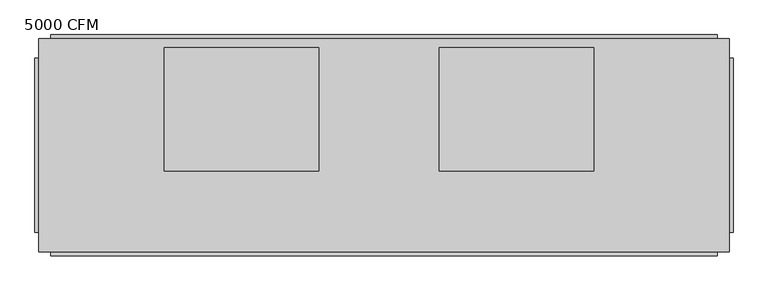
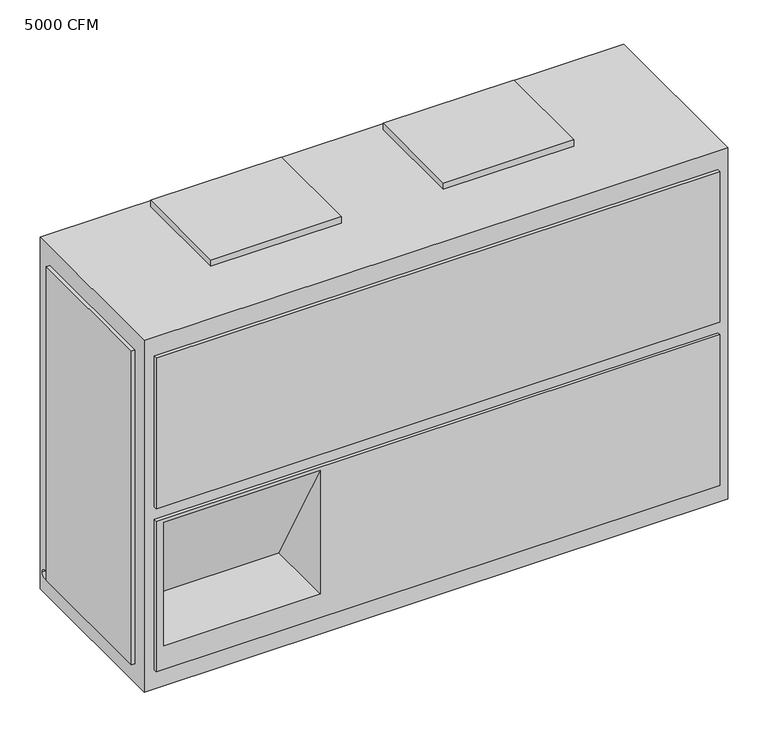
"""IFC4 building model written with IfcOpenShell, lengths in millimetres: proxy geometry, Air_Handling_Unit_-_Vertical_Packaged_-_DX_-_125-25_Tonsrfa_5458 : 5000 CFM."""

from ifc_helpers import new_model, si_unit, frame, origin, place, context, project, spatial, polyline, circle_curve, source, transform, mapped, element, save
from ifc_brep_helpers import plane_surface, revolved_surface, advanced_brep


def proxy_5000_cfm_f7311cc6(model_context):
    return source(origin(), model_context, "Body", "AdvancedBrep", [
        advanced_brep(
        [(2247.9, 703.2625, 1423.9875), (12.7, 703.2625, 1423.9875), (12.7, 12.7, 1423.9875), (2247.9, 12.7, 1423.9875), (419.1, 674.6875, 1423.9875), (919.1, 674.6875, 1423.9875), (919.1, 274.6875, 1423.9875), (419.1, 274.6875, 1423.9875), (1309.625, 674.6875, 1423.9875), (1809.625, 674.6875, 1423.9875), (1809.625, 274.6875, 1423.9875), (1309.625, 274.6875, 1423.9875), (2247.9, 703.2625, 0.0), (2247.9, 12.7, 0.0), (12.7, 12.7, 0.0), (12.7, 703.2625, 0.0), (2209.8, 703.2625, 686.59375), (50.8, 703.2625, 686.59375), (50.8, 703.2625, 76.2), (2209.8, 703.2625, 76.2), (2209.8, 703.2625, 1347.7875), (50.8, 703.2625, 1347.7875), (50.8, 703.2625, 737.39375), (2209.8, 703.2625, 737.39375), (12.7, 658.8125, 76.2), (12.7, 690.5625, 76.2), (12.7, 639.7625, 1347.7875), (12.7, 76.2, 1347.7875), (12.7, 76.2, 76.2), (12.7, 639.7625, 76.2), (50.8, 12.7, 686.59375), (2209.8, 12.7, 686.59375), (2209.8, 12.7, 76.2), (50.8, 12.7, 76.2), (50.8, 12.7, 1347.7875), (2209.8, 12.7, 1347.7875), (2209.8, 12.7, 737.39375), (50.8, 12.7, 737.39375), (2247.9, 696.9125, 280.9875), (2247.9, 652.4625, 280.9875), (2247.9, 688.975, 357.1875), (2247.9, 660.4, 357.1875), (2247.9, 688.975, 407.9875), (2247.9, 660.4, 407.9875), (2247.9, 696.9125, 484.1875), (2247.9, 652.4625, 484.1875), (2247.9, 685.8, 1128.7125), (2247.9, 663.575, 1128.7125), (2247.9, 76.2, 1347.7875), (2247.9, 639.7625, 1347.7875), (2247.9, 639.7625, 76.2), (2247.9, 76.2, 76.2), (2247.9, 685.8, 1090.6125), (2247.9, 663.575, 1090.6125), (50.8, 658.8125, 76.2), (50.8, 690.5625, 76.2), (2209.8, 696.9125, 280.9875), (2209.8, 652.4625, 280.9875), (2209.8, 660.4, 357.1875), (2209.8, 688.975, 357.1875), (2209.8, 660.4, 407.9875), (2209.8, 688.975, 407.9875), (2209.8, 652.4625, 484.1875), (2209.8, 696.9125, 484.1875), (2209.8, 663.575, 1128.7125), (2209.8, 685.8, 1128.7125), (0.0, 639.7625, 1347.7875), (0.0, 76.2, 1347.7875), (2260.6, 76.2, 1347.7875), (2260.6, 639.7625, 1347.7875), (2260.6, 639.7625, 76.2), (2260.6, 76.2, 76.2), (0.0, 76.2, 76.2), (0.0, 639.7625, 76.2), (2209.8, 715.9625, 686.59375), (50.8, 715.9625, 686.59375), (50.8, 0.0, 686.59375), (2209.8, 0.0, 686.59375), (2209.8, 0.0, 76.2), (50.8, 0.0, 76.2), (50.8, 715.9625, 76.2), (2209.8, 715.9625, 76.2), (679.375, 0.0, 671.45), (679.375, 0.0, 171.45), (79.375, 0.0, 171.45), (79.375, 0.0, 671.45), (679.375, 274.6875, 171.45), (79.375, 274.6875, 171.45), (2209.8, 715.9625, 1347.7875), (50.8, 715.9625, 1347.7875), (50.8, 0.0, 1347.7875), (2209.8, 0.0, 1347.7875), (2209.8, 0.0, 737.39375), (50.8, 0.0, 737.39375), (50.8, 715.9625, 737.39375), (2209.8, 715.9625, 737.39375), (919.1, 674.6875, 1449.3875), (419.1, 674.6875, 1449.3875), (419.1, 274.6875, 1449.3875), (919.1, 274.6875, 1449.3875), (1809.625, 674.6875, 1449.3875), (1309.625, 674.6875, 1449.3875), (1309.625, 274.6875, 1449.3875), (1809.625, 274.6875, 1449.3875), (2209.8, 663.575, 1090.6125), (2209.8, 685.8, 1090.6125)],
        [
            (0, 1),
            (1, 2),
            (2, 3),
            (3, 0),
            (4, 5),
            (5, 6),
            (6, 7),
            (7, 4),
            (8, 9),
            (9, 10),
            (10, 11),
            (11, 8),
            (12, 13),
            (13, 14),
            (14, 15),
            (15, 12),
            (0, 12),
            (15, 1),
            (16, 17),
            (17, 18),
            (18, 19),
            (19, 16),
            (20, 21),
            (21, 22),
            (22, 23),
            (23, 20),
            (14, 2),
            (24, 25, circle_curve(frame((12.7, 674.6875, 76.2), z_axis=(1.0, 0.0, 0.0), x_axis=(0.0, 1.0, 0.0)), 15.875)),
            (25, 24, circle_curve(frame((12.7, 674.6875, 76.2), z_axis=(1.0, 0.0, 0.0), x_axis=(0.0, 1.0, 0.0)), 15.875)),
            (26, 27),
            (27, 28),
            (28, 29),
            (29, 26),
            (13, 3),
            (30, 31),
            (31, 32),
            (32, 33),
            (33, 30),
            (34, 35),
            (35, 36),
            (36, 37),
            (37, 34),
            (38, 39, circle_curve(frame((2247.9, 674.6875, 280.9875), z_axis=(-1.0, 0.0, 0.0), x_axis=(0.0, 1.0, 0.0)), 22.225)),
            (39, 38, circle_curve(frame((2247.9, 674.6875, 280.9875), z_axis=(-1.0, 0.0, 0.0), x_axis=(0.0, 1.0, 0.0)), 22.225)),
            (40, 41, circle_curve(frame((2247.9, 674.6875, 357.1875), z_axis=(-1.0, 0.0, 0.0), x_axis=(0.0, 1.0, 0.0)), 14.2875)),
            (41, 40, circle_curve(frame((2247.9, 674.6875, 357.1875), z_axis=(-1.0, 0.0, 0.0), x_axis=(0.0, 1.0, 0.0)), 14.2875)),
            (42, 43, circle_curve(frame((2247.9, 674.6875, 407.9875), z_axis=(-1.0, 0.0, 0.0), x_axis=(0.0, 1.0, 0.0)), 14.2875)),
            (43, 42, circle_curve(frame((2247.9, 674.6875, 407.9875), z_axis=(-1.0, 0.0, 0.0), x_axis=(0.0, 1.0, 0.0)), 14.2875)),
            (44, 45, circle_curve(frame((2247.9, 674.6875, 484.1875), z_axis=(-1.0, 0.0, 0.0), x_axis=(0.0, 1.0, 0.0)), 22.225)),
            (45, 44, circle_curve(frame((2247.9, 674.6875, 484.1875), z_axis=(-1.0, 0.0, 0.0), x_axis=(0.0, 1.0, 0.0)), 22.225)),
            (46, 47, circle_curve(frame((2247.9, 674.6875, 1128.7125), z_axis=(-1.0, 0.0, 0.0), x_axis=(0.0, 1.0, 0.0)), 11.1125)),
            (47, 46, circle_curve(frame((2247.9, 674.6875, 1128.7125), z_axis=(-1.0, 0.0, 0.0), x_axis=(0.0, 1.0, 0.0)), 11.1125)),
            (48, 49),
            (49, 50),
            (50, 51),
            (51, 48),
            (52, 53, circle_curve(frame((2247.9, 674.6875, 1090.6125), z_axis=(-1.0, 0.0, 0.0), x_axis=(0.0, 1.0, 0.0)), 11.1125)),
            (53, 52, circle_curve(frame((2247.9, 674.6875, 1090.6125), z_axis=(-1.0, 0.0, 0.0), x_axis=(0.0, 1.0, 0.0)), 11.1125)),
            (54, 55, circle_curve(frame((50.8, 674.6875, 76.2), z_axis=(-1.0, 0.0, 0.0), x_axis=(0.0, 1.0, 0.0)), 15.875)),
            (55, 54, circle_curve(frame((50.8, 674.6875, 76.2), z_axis=(-1.0, 0.0, 0.0), x_axis=(0.0, 1.0, 0.0)), 15.875)),
            (55, 25),
            (24, 54),
            (38, 56),
            (56, 57, circle_curve(frame((2209.8, 674.6875, 280.9875), z_axis=(-1.0, 0.0, 0.0), x_axis=(0.0, 1.0, 0.0)), 22.225)),
            (57, 39),
            (57, 56, circle_curve(frame((2209.8, 674.6875, 280.9875), z_axis=(-1.0, 0.0, 0.0), x_axis=(0.0, 1.0, 0.0)), 22.225)),
            (58, 59, circle_curve(frame((2209.8, 674.6875, 357.1875), z_axis=(1.0, 0.0, 0.0), x_axis=(0.0, 1.0, 0.0)), 14.2875)),
            (59, 58, circle_curve(frame((2209.8, 674.6875, 357.1875), z_axis=(1.0, 0.0, 0.0), x_axis=(0.0, 1.0, 0.0)), 14.2875)),
            (58, 41),
            (40, 59),
            (60, 61, circle_curve(frame((2209.8, 674.6875, 407.9875), z_axis=(1.0, 0.0, 0.0), x_axis=(0.0, 1.0, 0.0)), 14.2875)),
            (61, 60, circle_curve(frame((2209.8, 674.6875, 407.9875), z_axis=(1.0, 0.0, 0.0), x_axis=(0.0, 1.0, 0.0)), 14.2875)),
            (60, 43),
            (42, 61),
            (62, 63, circle_curve(frame((2209.8, 674.6875, 484.1875), z_axis=(1.0, 0.0, 0.0), x_axis=(0.0, 1.0, 0.0)), 22.225)),
            (63, 62, circle_curve(frame((2209.8, 674.6875, 484.1875), z_axis=(1.0, 0.0, 0.0), x_axis=(0.0, 1.0, 0.0)), 22.225)),
            (62, 45),
            (44, 63),
            (64, 65, circle_curve(frame((2209.8, 674.6875, 1128.7125), z_axis=(1.0, 0.0, 0.0), x_axis=(0.0, 1.0, 0.0)), 11.1125)),
            (65, 64, circle_curve(frame((2209.8, 674.6875, 1128.7125), z_axis=(1.0, 0.0, 0.0), x_axis=(0.0, 1.0, 0.0)), 11.1125)),
            (64, 47),
            (46, 65),
            (66, 67),
            (67, 27),
            (26, 66),
            (68, 69),
            (69, 49),
            (48, 68),
            (70, 71),
            (71, 51),
            (50, 70),
            (72, 73),
            (73, 29),
            (28, 72),
            (69, 70),
            (73, 66),
            (72, 67),
            (71, 68),
            (74, 75),
            (75, 17),
            (16, 74),
            (76, 77),
            (77, 31),
            (30, 76),
            (78, 79),
            (79, 33),
            (32, 78),
            (80, 81),
            (81, 19),
            (18, 80),
            (74, 81),
            (80, 75),
            (79, 76),
            (78, 77),
            (82, 83),
            (83, 84),
            (84, 85),
            (85, 82),
            (86, 83),
            (82, 86),
            (87, 85),
            (84, 87),
            (87, 86),
            (88, 89),
            (89, 21),
            (20, 88),
            (90, 91),
            (91, 35),
            (34, 90),
            (92, 93),
            (93, 37),
            (36, 92),
            (94, 95),
            (95, 23),
            (22, 94),
            (88, 95),
            (94, 89),
            (93, 90),
            (92, 91),
            (96, 97),
            (97, 98),
            (98, 99),
            (99, 96),
            (96, 5),
            (4, 97),
            (7, 98),
            (6, 99),
            (100, 101),
            (101, 102),
            (102, 103),
            (103, 100),
            (100, 9),
            (8, 101),
            (11, 102),
            (10, 103),
            (104, 105, circle_curve(frame((2209.8, 674.6875, 1090.6125), z_axis=(1.0, 0.0, 0.0), x_axis=(0.0, 1.0, 0.0)), 11.1125)),
            (105, 104, circle_curve(frame((2209.8, 674.6875, 1090.6125), z_axis=(1.0, 0.0, 0.0), x_axis=(0.0, 1.0, 0.0)), 11.1125)),
            (104, 53),
            (52, 105),
        ],
        [
            plane_surface(frame((12.7, 703.2625, 1423.9875), z_axis=(0.0, 0.0, 1.0), x_axis=(-1.0, 0.0, 0.0))),
            plane_surface(frame((12.7, 703.2625, 0.0), z_axis=(0.0, 0.0, -1.0), x_axis=(1.0, 0.0, 0.0))),
            plane_surface(frame((2247.9, 703.2625, 1423.9875), z_axis=(0.0, 1.0, 0.0), x_axis=(0.0, 0.0, -1.0))),
            plane_surface(frame((12.7, 703.2625, 1423.9875), z_axis=(-1.0, 0.0, 0.0), x_axis=(0.0, 0.0, -1.0))),
            plane_surface(frame((12.7, 12.7, 1423.9875), z_axis=(0.0, -1.0, 0.0), x_axis=(0.0, 0.0, -1.0))),
            plane_surface(frame((2247.9, 12.7, 1423.9875), z_axis=(1.0, 0.0, 0.0), x_axis=(0.0, 0.0, -1.0))),
            plane_surface(frame((50.8, 690.5625, 76.2), z_axis=(-1.0, 0.0, 0.0), x_axis=(0.0, 0.0, 1.0))),
            revolved_surface(polyline([(50.8, 690.5625, 76.2), (12.7, 690.5625, 76.2)]), (12.7, 674.6875, 76.2), (1.0, 0.0, 0.0)),
            revolved_surface(polyline([(2247.9, 696.9125, 280.9875), (2209.8, 696.9125, 280.9875)]), (679.375, 674.6875, 280.9875), (1.0, 0.0, 0.0)),
            plane_surface(frame((2209.8, 688.975, 357.1875), z_axis=(1.0, 0.0, 0.0), x_axis=(0.0, 0.0, -1.0))),
            revolved_surface(polyline([(2247.9, 688.975, 357.1875), (2209.8, 688.975, 357.1875)]), (2209.8, 674.6875, 357.1875), (1.0, 0.0, 0.0)),
            plane_surface(frame((2209.8, 688.975, 407.9875), z_axis=(1.0, 0.0, 0.0), x_axis=(0.0, 0.0, -1.0))),
            revolved_surface(polyline([(2247.9, 688.975, 407.9875), (2209.8, 688.975, 407.9875)]), (2209.8, 674.6875, 407.9875), (1.0, 0.0, 0.0)),
            plane_surface(frame((2209.8, 696.9125, 484.1875), z_axis=(1.0, 0.0, 0.0), x_axis=(0.0, 0.0, -1.0))),
            revolved_surface(polyline([(2247.9, 696.9125, 484.1875), (2209.8, 696.9125, 484.1875)]), (2209.8, 674.6875, 484.1875), (1.0, 0.0, 0.0)),
            plane_surface(frame((2209.8, 685.8, 1128.7125), z_axis=(1.0, 0.0, 0.0), x_axis=(0.0, 0.0, -1.0))),
            revolved_surface(polyline([(2247.9, 685.8, 1128.7125), (2209.8, 685.8, 1128.7125)]), (2209.8, 674.6875, 1128.7125), (1.0, 0.0, 0.0)),
            plane_surface(frame((0.0, 639.7625, 1347.7875), z_axis=(0.0, 0.0, 1.0), x_axis=(-1.0, 0.0, 0.0))),
            plane_surface(frame((0.0, 639.7625, 76.2), z_axis=(0.0, 0.0, -1.0), x_axis=(1.0, 0.0, 0.0))),
            plane_surface(frame((2260.6, 639.7625, 1347.7875), z_axis=(0.0, 1.0, 0.0), x_axis=(0.0, 0.0, -1.0))),
            plane_surface(frame((0.0, 639.7625, 1347.7875), z_axis=(-1.0, 0.0, 0.0), x_axis=(0.0, 0.0, -1.0))),
            plane_surface(frame((0.0, 76.2, 1347.7875), z_axis=(0.0, -1.0, 0.0), x_axis=(0.0, 0.0, -1.0))),
            plane_surface(frame((2260.6, 76.2, 1347.7875), z_axis=(1.0, 0.0, 0.0), x_axis=(0.0, 0.0, -1.0))),
            plane_surface(frame((50.8, 715.9625, 686.59375), z_axis=(0.0, 0.0, 1.0), x_axis=(-1.0, 0.0, 0.0))),
            plane_surface(frame((50.8, 715.9625, 76.2), z_axis=(0.0, 0.0, -1.0), x_axis=(1.0, 0.0, 0.0))),
            plane_surface(frame((2209.8, 715.9625, 686.59375), z_axis=(0.0, 1.0, 0.0), x_axis=(0.0, 0.0, -1.0))),
            plane_surface(frame((50.8, 715.9625, 686.59375), z_axis=(-1.0, 0.0, 0.0), x_axis=(0.0, 0.0, -1.0))),
            plane_surface(frame((50.8, 0.0, 686.59375), z_axis=(0.0, -1.0, 0.0), x_axis=(0.0, 0.0, -1.0))),
            plane_surface(frame((2209.8, 0.0, 686.59375), z_axis=(1.0, 0.0, 0.0), x_axis=(0.0, 0.0, -1.0))),
            plane_surface(frame((679.375, 0.0, 671.45), z_axis=(-1.0, 0.0, 0.0), x_axis=(0.0, -0.4814981342249409, 0.8764471157679172))),
            plane_surface(frame((79.375, 0.0, 671.45), z_axis=(1.0, 0.0, 0.0), x_axis=(0.0, 0.4814981342249409, -0.8764471157679172))),
            plane_surface(frame((679.375, 274.6875, 171.45), z_axis=(0.0, -0.8764471157679172, -0.4814981342249409), x_axis=(-1.0, 0.0, 0.0))),
            plane_surface(frame((679.375, 0.0, 171.45), z_axis=(0.0, 0.0, 1.0), x_axis=(-1.0, 0.0, 0.0))),
            plane_surface(frame((50.8, 715.9625, 1347.7875), z_axis=(0.0, 0.0, 1.0), x_axis=(-1.0, 0.0, 0.0))),
            plane_surface(frame((50.8, 715.9625, 737.39375), z_axis=(0.0, 0.0, -1.0), x_axis=(1.0, 0.0, 0.0))),
            plane_surface(frame((2209.8, 715.9625, 1347.7875), z_axis=(0.0, 1.0, 0.0), x_axis=(0.0, 0.0, -1.0))),
            plane_surface(frame((50.8, 715.9625, 1347.7875), z_axis=(-1.0, 0.0, 0.0), x_axis=(0.0, 0.0, -1.0))),
            plane_surface(frame((50.8, 0.0, 1347.7875), z_axis=(0.0, -1.0, 0.0), x_axis=(0.0, 0.0, -1.0))),
            plane_surface(frame((2209.8, 0.0, 1347.7875), z_axis=(1.0, 0.0, 0.0), x_axis=(0.0, 0.0, -1.0))),
            plane_surface(frame((419.1, 674.6875, 1449.3875), z_axis=(0.0, 0.0, 1.0), x_axis=(-1.0, 0.0, 0.0))),
            plane_surface(frame((919.1, 674.6875, 1449.3875), z_axis=(0.0, 1.0, 0.0), x_axis=(0.0, 0.0, -1.0))),
            plane_surface(frame((419.1, 674.6875, 1449.3875), z_axis=(-1.0, 0.0, 0.0), x_axis=(0.0, 0.0, -1.0))),
            plane_surface(frame((419.1, 274.6875, 1449.3875), z_axis=(0.0, -1.0, 0.0), x_axis=(0.0, 0.0, -1.0))),
            plane_surface(frame((919.1, 274.6875, 1449.3875), z_axis=(1.0, 0.0, 0.0), x_axis=(0.0, 0.0, -1.0))),
            plane_surface(frame((1309.625, 674.6875, 1449.3875), z_axis=(0.0, 0.0, 1.0), x_axis=(-1.0, 0.0, 0.0))),
            plane_surface(frame((1809.625, 674.6875, 1449.3875), z_axis=(0.0, 1.0, 0.0), x_axis=(0.0, 0.0, -1.0))),
            plane_surface(frame((1309.625, 674.6875, 1449.3875), z_axis=(-1.0, 0.0, 0.0), x_axis=(0.0, 0.0, -1.0))),
            plane_surface(frame((1309.625, 274.6875, 1449.3875), z_axis=(0.0, -1.0, 0.0), x_axis=(0.0, 0.0, -1.0))),
            plane_surface(frame((1809.625, 274.6875, 1449.3875), z_axis=(1.0, 0.0, 0.0), x_axis=(0.0, 0.0, -1.0))),
            plane_surface(frame((2209.8, 685.8, 1090.6125), z_axis=(1.0, 0.0, 0.0), x_axis=(0.0, 0.0, -1.0))),
            revolved_surface(polyline([(2247.9, 685.8, 1090.6125), (2209.8, 685.8, 1090.6125)]), (2209.8, 674.6875, 1090.6125), (1.0, 0.0, 0.0)),
        ],
        [
            (0, [[1, 2, 3, 4], [5, 6, 7, 8], [9, 10, 11, 12]]),
            (1, [[13, 14, 15, 16]]),
            (2, [[-1, 17, -16, 18], [19, 20, 21, 22], [23, 24, 25, 26]]),
            (3, [[-2, -18, -15, 27], [28, 29], [30, 31, 32, 33]]),
            (4, [[-3, -27, -14, 34], [35, 36, 37, 38], [39, 40, 41, 42]]),
            (5, [[-4, -34, -13, -17], [43, 44], [45, 46], [47, 48], [49, 50], [51, 52], [53, 54, 55, 56], [57, 58]]),
            (6, [[59, 60]]),
            (7, [[-60, 61, -28, 62]]),
            (7, [[-59, -62, -29, -61]]),
            (8, [[-43, 63, 64, 65]]),
            (8, [[-44, -65, 66, -63]]),
            (9, [[67, 68]]),
            (10, [[-67, 69, -45, 70]]),
            (10, [[-68, -70, -46, -69]]),
            (11, [[71, 72]]),
            (12, [[-71, 73, -47, 74]]),
            (12, [[-72, -74, -48, -73]]),
            (13, [[75, 76]]),
            (14, [[-75, 77, -49, 78]]),
            (14, [[-76, -78, -50, -77]]),
            (15, [[79, 80]]),
            (16, [[-79, 81, -51, 82]]),
            (16, [[-80, -82, -52, -81]]),
            (17, [[83, 84, -30, 85]]),
            (17, [[86, 87, -53, 88]]),
            (18, [[89, 90, -55, 91]]),
            (18, [[92, 93, -32, 94]]),
            (19, [[95, -91, -54, -87]]),
            (19, [[96, -85, -33, -93]]),
            (20, [[-83, -96, -92, 97]]),
            (21, [[-97, -94, -31, -84]]),
            (21, [[98, -88, -56, -90]]),
            (22, [[-86, -98, -89, -95]]),
            (23, [[99, 100, -19, 101]]),
            (23, [[102, 103, -35, 104]]),
            (24, [[105, 106, -37, 107]]),
            (24, [[108, 109, -21, 110]]),
            (25, [[-99, 111, -108, 112]]),
            (26, [[-112, -110, -20, -100]]),
            (26, [[113, -104, -38, -106]]),
            (27, [[-102, -113, -105, 114], [115, 116, 117, 118]]),
            (28, [[-64, -66]]),
            (28, [[-111, -101, -22, -109]]),
            (28, [[-114, -107, -36, -103]]),
            (29, [[119, -115, 120]]),
            (30, [[121, -117, 122]]),
            (31, [[-120, -118, -121, 123]]),
            (32, [[-119, -123, -122, -116]]),
            (33, [[124, 125, -23, 126]]),
            (33, [[127, 128, -39, 129]]),
            (34, [[130, 131, -41, 132]]),
            (34, [[133, 134, -25, 135]]),
            (35, [[-124, 136, -133, 137]]),
            (36, [[-137, -135, -24, -125]]),
            (36, [[138, -129, -42, -131]]),
            (37, [[-127, -138, -130, 139]]),
            (38, [[-136, -126, -26, -134]]),
            (38, [[-139, -132, -40, -128]]),
            (39, [[140, 141, 142, 143]]),
            (40, [[-140, 144, -5, 145]]),
            (41, [[-141, -145, -8, 146]]),
            (42, [[-142, -146, -7, 147]]),
            (43, [[-143, -147, -6, -144]]),
            (44, [[148, 149, 150, 151]]),
            (45, [[-148, 152, -9, 153]]),
            (46, [[-149, -153, -12, 154]]),
            (47, [[-150, -154, -11, 155]]),
            (48, [[-151, -155, -10, -152]]),
            (49, [[156, 157]]),
            (50, [[-156, 158, -57, 159]]),
            (50, [[-157, -159, -58, -158]]),
        ],
    ),
    ])


if __name__ == "__main__":
    model = new_model("IFC4")
    model_context = context("Model", 3, world=origin())
    ifc_project = project(units=[si_unit("LENGTHUNIT", "METRE", prefix="MILLI")], contexts=[model_context])
    site = spatial("IfcSite", under=ifc_project)
    building = spatial("IfcBuilding", under=site)
    placement = place(None, origin())
    proxy_5000_cfm_shape = proxy_5000_cfm_f7311cc6(model_context)
    element("IfcBuildingElementProxy", 1, Name="Air_Handling_Unit_-_Vertical_Packaged_-_DX_-_125-25_Tonsrfa_5458 : 5000 CFM", ObjectType="Air_Handling_Unit_-_Vertical_Packaged_-_DX_-_125-25_Tonsrfa_5458 : 5000 CFM", at=placement, inside=building, context=model_context, shape_type="MappedRepresentation", body=[
        mapped(proxy_5000_cfm_shape, transform((0.0, 0.0, 0.0), x_axis=(1.0, 0.0, 0.0), y_axis=(0.0, 1.0, 0.0), z_axis=(0.0, 0.0, 1.0))),
    ])
    save(model, "model.ifc")

# Revit data of these elements
# Type "Air_Handling_Unit_-_Vertical_Packaged_-_DX_-_125-25_Tonsrfa_5458 : 5000 CFM"
#   Model = "ART654657"
#   Manufacturer = "AIRHandlers LTD"
#   Description = "Air Handeling Unit"
#   COBie.Type.CreatedBy = "design@eagle.com"
#   COBie.Type.CreatedOn = "2016-09-13T05:47:35"
#   COBie.Type.Name = "Mechanical Equipment_Air_Handling_Unit_-_Vertical_Packaged_-_DX_-_125-25_Tonsrfa_5458_5000 CFM"
#   COBie.Type.Category = "23-75 35 14 21 : Modular Rooftop Air Handling Units"
#   COBie.Type.Description = "Air Handeling Unit"
#   COBie.Type.Manufacturer = "AIRHandlers LTD"
#   COBie.Type.ModelNumber = "ART654657"
#   Operating Charge [instance default] = "4.0 lb"
#   COBie.Type.ReplacementCost = 0
#   Working Pressure [instance default] = 2999219.3 Pa
#   Voltage = 400 V
#   Supply Air Outlet Width = 500 mm
#   Supply Air Outlet Height = 400 mm
#   Return Air Inlet Width = 600 mm
#   Return Air Inlet Height = 500 mm
#   Power Wire Radius = 11.113 mm
#   Power Wire Diameter = 22.225 mm
#   Outlet Radius = 22.225 mm
#   Outlet Diameter = 44.45 mm
#   Nominal Capacity [instance default] = 43960.7 W
#   Inlet Radius = 14.288 mm
#   Inlet Diameter = 28.575 mm
#   External Static Pressure [instance default] = 497.68 Pa
#   Drain Radius = 15.875 mm
#   Drain Flow [instance default] = 0.0 L/s
#   Drain Diameter = 31.75 mm
#   Distance = 390.525 mm
#   Control Wire Radius = 11.113 mm
#   Control Wire Diameter = 22.225 mm
#   C9 Offset 1 = 1090.612 mm
#   Apparent Load = 4560 VA
#   Air Flow = 2359.74 L/s
#   AHU Width = 715.963 mm
#   AHU Length = 2260.6 mm
#   AHU Height = 1423.987 mm
#   COBie.Type = yes
#   Number of Poles = 3
#   AHU Material = none
